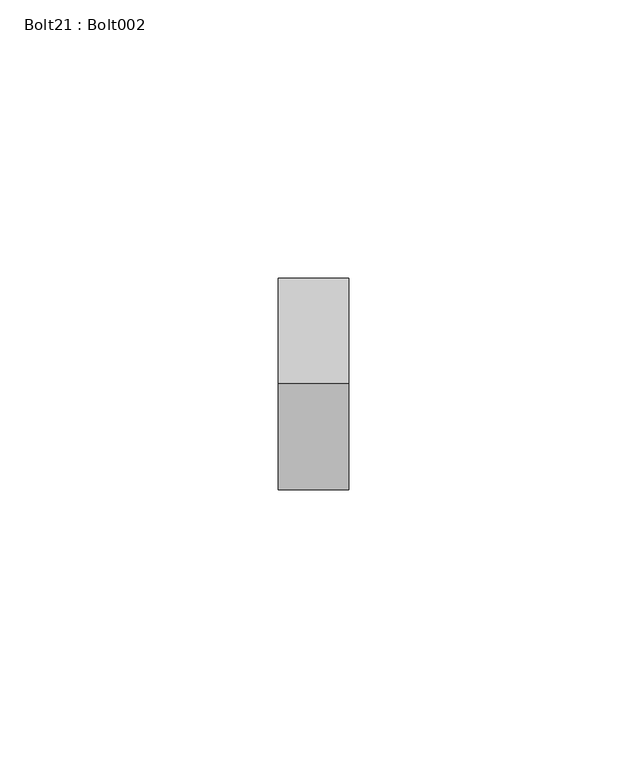
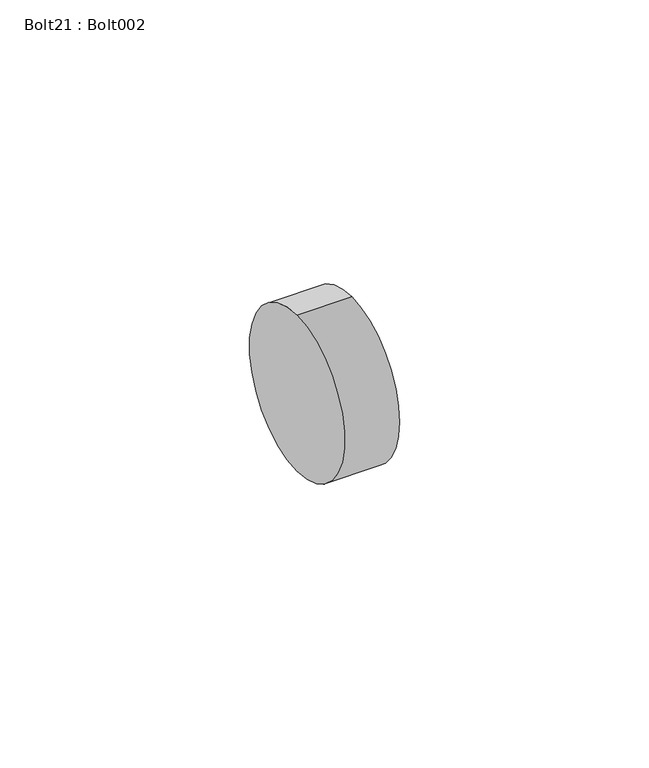
"""IFC4 building model written with IfcOpenShell, lengths in millimetres: proxy geometry, Bolt21 : Bolt002."""

from ifc_helpers import new_model, si_unit, point, frame, frame_2d, origin, place, context, project, spatial, circle_curve, trimmed, segment, composite_curve, outline, extrude, source, transform, mapped, element, save


def bolt21_bolt002_beea302d(model_context):
    return source(origin(), model_context, "Body", "SweptSolid", [
        extrude(outline(composite_curve([segment(trimmed(circle_curve(frame_2d((1985.8304801, 40070.0545241)), 19.05), [point((1985.8304801, 40051.0045241))], [point((1985.8304801, 40089.1045241))], False, "CARTESIAN"), True, "CONTINUOUS"), segment(trimmed(circle_curve(frame_2d((1985.8304801, 40070.0545241)), 19.05), [point((1985.8304801, 40089.1045241))], [point((1985.8304801, 40051.0045241))], False, "CARTESIAN"), True, "CONTINUOUS")], self_intersect=False)), frame((10268.2640809, 0.0, 0.0), z_axis=(1.0, 0.0, 0.0), x_axis=(0.0, 1.0, 0.0)), (0.0, 0.0, 1.0), 12.7),
    ])


if __name__ == "__main__":
    model = new_model("IFC4")
    model_context = context("Model", 3, world=origin())
    ifc_project = project(units=[si_unit("LENGTHUNIT", "METRE", prefix="MILLI")], contexts=[model_context])
    site = spatial("IfcSite", under=ifc_project)
    building = spatial("IfcBuilding", under=site)
    placement = place(None, origin())
    bolt21_bolt002_shape = bolt21_bolt002_beea302d(model_context)
    element("IfcBuildingElementProxy", 1, Name="Bolt21 : Bolt002", ObjectType="Bolt21 : Bolt002", at=placement, inside=building, context=model_context, shape_type="MappedRepresentation", body=[
        mapped(bolt21_bolt002_shape, transform((0.0, 0.0, 0.0), x_axis=(1.0, 0.0, 0.0), y_axis=(0.0, 1.0, 0.0), z_axis=(0.0, 0.0, 1.0))),
    ])
    save(model, "model.ifc")

# Revit data of these elements
# Type "Bolt21 : Bolt002"
#   NameOverride = "Bolt002"
# Element 1 (IfcBuildingElementProxy, "Bolt21 : Bolt002")
#   Materials on its faces: "TUBE STEEL STRINGER WELDED TO ANCHORED STEEL PLATE - SEE STRUCT DWGS"
# Materials
#   "TUBE STEEL STRINGER WELDED TO ANCHORED STEEL PLATE - SEE STRUCT DWGS": class "Unassigned", colour RGB 128 128 128, transparency 0, Cost = 0
